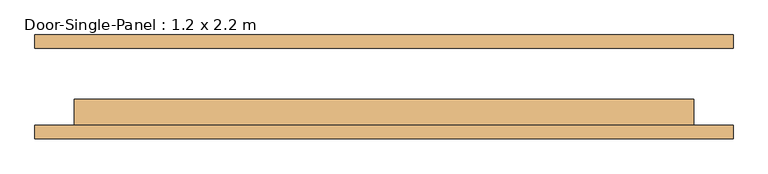
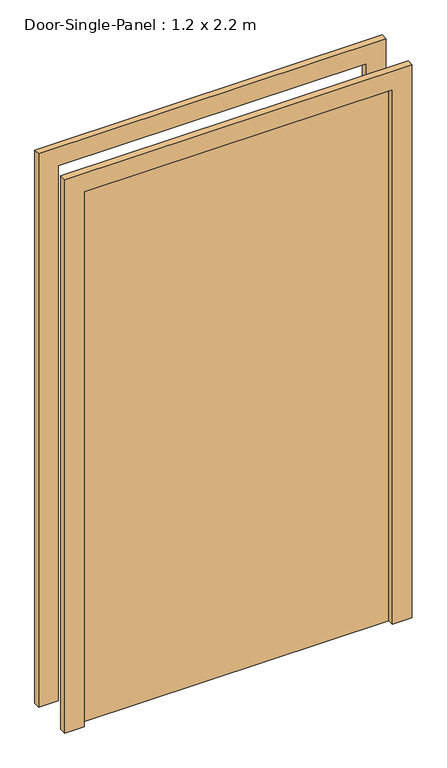
"""IFC4 building model written with IfcOpenShell, lengths in millimetres: door geometry, Door-Single-Panel : 1.2 x 2.2 m."""

from ifc_helpers import new_model, si_unit, frame, origin, origin_with_axes, place, context, project, spatial, polyline, outline, extrude, source, transform, mapped, element, save


def door_single_panel_1_2_x_2_2_m_3fbad9d7(model_context):
    return source(origin(), model_context, "Body", "SweptSolid", [
        extrude(outline(polyline([(600.0, -24.2), (600.0, -75.0), (-600.0, -75.0), (-600.0, -24.2), (600.0, -24.2)])), origin_with_axes(), (0.0, 0.0, 1.0), 2200.0),
        extrude(outline(polyline([(2276.2, 676.2), (2276.2, -676.2), (0.0, -676.2), (0.0, -600.0), (2200.0, -600.0), (2200.0, 600.0), (0.0, 600.0), (0.0, 676.2), (2276.2, 676.2)])), frame((0.0, 75.0, 0.0), z_axis=(0.0, 1.0, 0.0), x_axis=(0.0, 0.0, 1.0)), (0.0, 0.0, 1.0), 25.4),
        extrude(outline(polyline([(2276.2, -676.2), (0.0, -676.2), (0.0, -600.0), (2200.0, -600.0), (2200.0, 600.0), (0.0, 600.0), (0.0, 676.2), (2276.2, 676.2), (2276.2, -676.2)])), frame((0.0, -100.4, 0.0), z_axis=(0.0, 1.0, 0.0), x_axis=(0.0, 0.0, 1.0)), (0.0, 0.0, 1.0), 25.4),
    ])


if __name__ == "__main__":
    model = new_model("IFC4")
    model_context = context("Model", 3, world=origin())
    ifc_project = project(units=[si_unit("LENGTHUNIT", "METRE", prefix="MILLI")], contexts=[model_context])
    site = spatial("IfcSite", under=ifc_project)
    building = spatial("IfcBuilding", under=site)
    placement = place(None, origin())
    door_single_panel_1_2_x_2_2_m_shape = door_single_panel_1_2_x_2_2_m_3fbad9d7(model_context)
    element("IfcDoor", 1, ObjectType="Door-Single-Panel : 1.2 x 2.2 m", at=placement, inside=building, context=model_context, shape_type="MappedRepresentation", body=[
        mapped(door_single_panel_1_2_x_2_2_m_shape, transform((0.0, 0.0, 0.0), x_axis=(1.0, 0.0, 0.0), y_axis=(0.0, 1.0, 0.0), z_axis=(0.0, 0.0, 1.0))),
    ])
    save(model, "model.ifc")

# Revit data of these elements
# Type "Door-Single-Panel : 1.2 x 2.2 m"
#   Type Mark = "47"
#   Construction Type Id = "DOOR"
#   Analytic Construction = "Wooden"
#   Thickness = 0.0508 m
#   Thermal Resistance (R) = 0.455703 (m²·K)/W
#   Swing Angle [instance default] = 90.00°
#   Heat Transfer Coefficient (U) = 2.19465 W/(m²·K)
#   Height = 2.2 m
#   Trim Projection Ext = 0.0254 m
#   Trim Projection Int = 0.0254 m
#   Trim Width = 0.0762 m
#   Width = 1.2 m
#   Define Thermal Properties by = 1
#   Panel Material = Wood - Birch - Solid Stained Light Low Gloss
#   Trim Material = Paint - Sienna
#   Visual Light Transmittance = 0
#   Solar Heat Gain Coefficient = 0
#   Function = (empty or 0)
#   Wall Closure = (empty or 0)
# Element 1 (IfcDoor, "Door-Single-Panel : 1.2 x 2.2 m")
#   Materials on its faces: "Paint - Sienna", "Wood - Birch - Solid Stained Light Low Gloss"
# Materials
#   "Wood - Birch - Solid Stained Light Low Gloss": class "Wood", colour RGB 210 159 95, transparency 0, Cost = 0
#   "Paint - Sienna": class "Miscellaneous", colour RGB 118 70 51, transparency 0, Cost = 0
